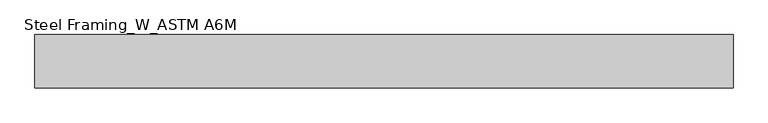
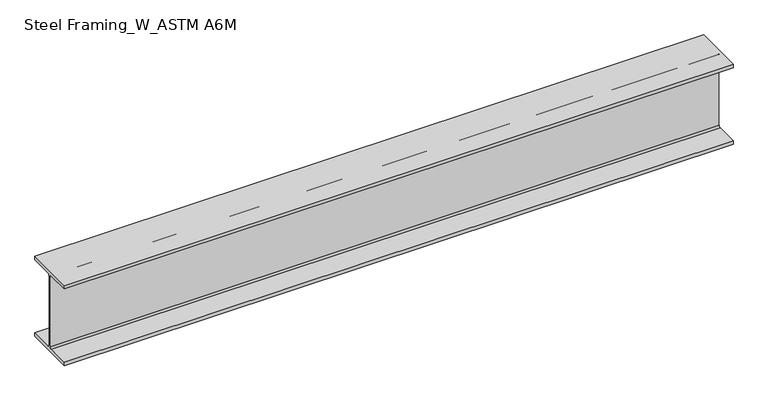
"""IFC4 building model written with IfcOpenShell, lengths in millimetres: beam geometry, Steel Framing_W_ASTM A6M : H_SB_AR_S02_W460x128_B1."""

import ifcopenshell
import ifcopenshell.guid

model = None  # the IFC model being written
_history = None  # IfcOwnerHistory: only IFC2X3 demands one
_inside = {}  # id of a spatial element -> (the spatial element, [elements in it])
_under = {}  # id of a project, library or spatial element -> (it, [spatial elements below it])
_declared = {}  # id of a project -> (the project, [libraries it declares])
_typed = {}  # id of a type object -> (the type object, [elements of that type])
_made_of = {}  # id of a material, layer set ... -> (it, [elements and type objects made of it])


def new_model(schema):
    """Start an empty IFC model of exactly this schema.

    Asked for "IFC4X3", IfcOpenShell would pick the latest addendum, in which some entities
    have other attributes; the version numbers below select the first issue.
    IFC2X3 requires an IfcOwnerHistory on every rooted entity: one is made here for all.
    """
    global model, _history
    if schema == "IFC4X3":
        model = ifcopenshell.file(schema_version=(4, 3, 0, 0))
    else:
        model = ifcopenshell.file(schema=schema)
    _inside.clear()
    _under.clear()
    _declared.clear()
    _typed.clear()
    _made_of.clear()
    _history = None
    if model.schema == "IFC2X3":
        org = make("IfcOrganization", Name="unknown")
        user = make(
            "IfcPersonAndOrganization",
            ThePerson=make("IfcPerson", FamilyName="unknown"),
            TheOrganization=org,
        )
        app = make(
            "IfcApplication",
            ApplicationDeveloper=org,
            Version="unknown",
            ApplicationFullName="unknown",
            ApplicationIdentifier="unknown",
        )
        _history = make(
            "IfcOwnerHistory",
            OwningUser=user,
            OwningApplication=app,
            ChangeAction="ADDED",
            CreationDate=0,
        )
    return model


def make(cls, **values):
    """One entity of the class cls with the attributes given. An attribute that is None is left unset."""
    return model.create_entity(
        cls, **{name: value for name, value in values.items() if value is not None}
    )


def rooted(cls, **values):
    """An entity with a GlobalId (a new one), such as an element, a storey or a relation."""
    return make(cls, GlobalId=ifcopenshell.guid.new(), OwnerHistory=_history, **values)


def si_unit(unit_type, name, prefix=None):
    """IfcSIUnit, for example si_unit("LENGTHUNIT", "METRE", prefix="MILLI")."""
    return make("IfcSIUnit", UnitType=unit_type, Prefix=prefix, Name=name)


def assignment(units):
    """IfcUnitAssignment: the units of a project."""
    return None if units is None else make("IfcUnitAssignment", Units=units)


def point(xyz):
    """IfcCartesianPoint."""
    return None if xyz is None else make("IfcCartesianPoint", Coordinates=xyz)


def direction(xyz):
    """IfcDirection."""
    return None if xyz is None else make("IfcDirection", DirectionRatios=xyz)


def frame(location, z_axis=None, x_axis=None):
    """IfcAxis2Placement3D, a coordinate frame: its origin and axes. An axis left out is left unset."""
    return make(
        "IfcAxis2Placement3D",
        Location=point(location),
        Axis=direction(z_axis),
        RefDirection=direction(x_axis),
    )


def frame_2d(location, x_axis=None):
    """IfcAxis2Placement2D, a coordinate frame in the plane: its origin and x axis."""
    return make(
        "IfcAxis2Placement2D", Location=point(location), RefDirection=direction(x_axis)
    )


def origin():
    """The frame at (0, 0, 0) with its axes left unset."""
    return frame((0.0, 0.0, 0.0))


def place(relative_to, where):
    """IfcLocalPlacement: puts the frame where relative to a parent placement (None: the world)."""
    return make(
        "IfcLocalPlacement", PlacementRelTo=relative_to, RelativePlacement=where
    )


def context(
    kind, dimensions, precision=None, world=None, true_north=None, identifier=None
):
    """IfcGeometricRepresentationContext, for example the 3D "Model" context."""
    return make(
        "IfcGeometricRepresentationContext",
        ContextIdentifier=identifier,
        ContextType=kind,
        CoordinateSpaceDimension=dimensions,
        Precision=precision,
        WorldCoordinateSystem=world,
        TrueNorth=true_north,
    )


def project(units=None, contexts=None):
    """IfcProject with its units and contexts."""
    return rooted(
        "IfcProject",
        Name="project",
        RepresentationContexts=contexts,
        UnitsInContext=assignment(units),
    )


def spatial(cls, under=None, at=None, **own):
    """A site, building, storey or space (cls), placed at a placement, below another one or the project."""
    s = rooted(cls, ObjectPlacement=at, **own)
    if under is not None:
        _under.setdefault(under.id(), (under, []))[1].append(s)
    return s


def polyline(points):
    """IfcPolyline through the points."""
    return make("IfcPolyline", Points=[point(p) for p in points])


def circle_curve(where, radius):
    """IfcCircle in the frame where."""
    return make("IfcCircle", Position=where, Radius=radius)


def trimmed(basis, trim1, trim2, sense, master):
    """IfcTrimmedCurve: the piece of a basis curve between two trims."""
    return make(
        "IfcTrimmedCurve",
        BasisCurve=basis,
        Trim1=trim1,
        Trim2=trim2,
        SenseAgreement=sense,
        MasterRepresentation=master,
    )


def segment(curve, same_sense, transition):
    """IfcCompositeCurveSegment."""
    return make(
        "IfcCompositeCurveSegment",
        Transition=transition,
        SameSense=same_sense,
        ParentCurve=curve,
    )


def composite_curve(segments, self_intersect=None):
    """IfcCompositeCurve: segments joined end to end."""
    return make("IfcCompositeCurve", Segments=segments, SelfIntersect=self_intersect)


def outline(outer, holes=None, kind="AREA"):
    """IfcArbitraryClosedProfileDef: a profile drawn as a closed curve; with holes, ...WithVoids."""
    if holes is None:
        return make("IfcArbitraryClosedProfileDef", ProfileType=kind, OuterCurve=outer)
    return make(
        "IfcArbitraryProfileDefWithVoids",
        ProfileType=kind,
        OuterCurve=outer,
        InnerCurves=holes,
    )


def extrude(swept, where, along, depth):
    """IfcExtrudedAreaSolid: the profile swept, set in the frame where, extruded along a direction by depth."""
    return make(
        "IfcExtrudedAreaSolid",
        SweptArea=swept,
        Position=where,
        ExtrudedDirection=direction(along),
        Depth=depth,
    )


def shape(context_of_items, identifier, shape_type, items):
    """IfcShapeRepresentation: the items that make up one representation, for example the "Body"."""
    return make(
        "IfcShapeRepresentation",
        ContextOfItems=context_of_items,
        RepresentationIdentifier=identifier,
        RepresentationType=shape_type,
        Items=items,
    )


def source(mapping_origin, context_of_items, identifier, shape_type, items):
    """IfcRepresentationMap: a shape defined once, which mapped items show again and again."""
    return make(
        "IfcRepresentationMap",
        MappingOrigin=mapping_origin,
        MappedRepresentation=shape(context_of_items, identifier, shape_type, items),
    )


def transform(
    local_origin,
    x_axis=None,
    y_axis=None,
    z_axis=None,
    scale=None,
    scale2=None,
    scale3=None,
    uniform=True,
):
    """IfcCartesianTransformationOperator3D, or its non-uniform kind. x_axis, y_axis, z_axis: its Axis1, 2, 3."""
    if uniform:
        return make(
            "IfcCartesianTransformationOperator3D",
            Axis1=direction(x_axis),
            Axis2=direction(y_axis),
            LocalOrigin=point(local_origin),
            Scale=scale,
            Axis3=direction(z_axis),
        )
    return make(
        "IfcCartesianTransformationOperator3DnonUniform",
        Axis1=direction(x_axis),
        Axis2=direction(y_axis),
        LocalOrigin=point(local_origin),
        Scale=scale,
        Axis3=direction(z_axis),
        Scale2=scale2,
        Scale3=scale3,
    )


def mapped(mapping_source, mapping_target):
    """IfcMappedItem: shows the shape of a source again, moved by a transform."""
    return make(
        "IfcMappedItem", MappingSource=mapping_source, MappingTarget=mapping_target
    )


def made_of(thing, what):
    """Note that an element or type object is made of a material, layer set ...; save() writes the relation."""
    if what is not None:
        _made_of.setdefault(what.id(), (what, []))[1].append(thing)
    return thing


def element(
    cls,
    number,
    at=None,
    inside=None,
    cuts=None,
    type_object=None,
    material=None,
    context=None,
    identifier="Body",
    shape_type=None,
    held_by="IfcProductDefinitionShape",
    body=None,
    shapes=None,
    **own,
):
    """One element of the class cls, such as IfcWall. Its Tag is "e" and its number.

    at: its placement. inside: the storey or other place that contains it. cuts: it is an
    opening in that element (IfcRelVoidsElement). A single representation is given by context,
    identifier, shape_type and body (its items); several are given by shapes. held_by: the class
    of the entity that holds the representations. save() writes the other relations.
    """
    e = rooted(cls, Tag="e%d" % number, ObjectPlacement=at, **own)
    if body is not None:
        shapes = [shape(context, identifier, shape_type, body)]
    if shapes is not None:
        e.Representation = make(held_by, Representations=shapes)
    if inside is not None:
        _inside.setdefault(inside.id(), (inside, []))[1].append(e)
    if cuts is not None:
        rooted(
            "IfcRelVoidsElement", RelatingBuildingElement=cuts, RelatedOpeningElement=e
        )
    if type_object is not None:
        _typed.setdefault(type_object.id(), (type_object, []))[1].append(e)
    return made_of(e, material)


def aggregate(whole, parts):
    """IfcRelAggregates: a whole, such as a stair, and the parts it consists of."""
    return rooted("IfcRelAggregates", RelatingObject=whole, RelatedObjects=parts)


def save(model, path):
    """Write the relations noted so far, then the file.

    IfcRelAggregates (storeys below a building ...), IfcRelContainedInSpatialStructure (elements
    in a storey), IfcRelDefinesByType, IfcRelAssociatesMaterial and IfcRelDeclares: one each for
    every whole, place, type object, material and project.
    """
    for whole, parts in _under.values():
        aggregate(whole, parts)
    for where, things in _inside.values():
        rooted(
            "IfcRelContainedInSpatialStructure",
            RelatedElements=things,
            RelatingStructure=where,
        )
    for kind, things in _typed.values():
        rooted("IfcRelDefinesByType", RelatedObjects=things, RelatingType=kind)
    for what, things in _made_of.values():
        rooted("IfcRelAssociatesMaterial", RelatedObjects=things, RelatingMaterial=what)
    for by, libraries in _declared.values():
        rooted("IfcRelDeclares", RelatingContext=by, RelatedDefinitions=libraries)
    model.write(path)


def steel_framing_w_astm_a6m_196e06da(model_context):
    return source(origin(), model_context, "Body", "SweptSolid", [
        extrude(outline(composite_curve([segment(polyline([(141.0, -213.9), (141.0, -233.5), (-141.0, -233.5), (-141.0, -213.9), (-16.2, -213.9)]), True, "CONTINUOUS"), segment(trimmed(circle_curve(frame_2d((-16.2, -203.8)), 10.1), [point((-16.2, -213.9))], [point((-6.1, -203.8))], True, "CARTESIAN"), True, "CONTINUOUS"), segment(polyline([(-6.1, -203.8), (-6.1, 203.8)]), True, "CONTINUOUS"), segment(trimmed(circle_curve(frame_2d((-16.2, 203.8)), 10.1), [point((-6.1, 203.8))], [point((-16.2, 213.9))], True, "CARTESIAN"), True, "CONTINUOUS"), segment(polyline([(-16.2, 213.9), (-141.0, 213.9), (-141.0, 233.5), (141.0, 233.5), (141.0, 213.9), (16.2, 213.9)]), True, "CONTINUOUS"), segment(trimmed(circle_curve(frame_2d((16.2, 203.8)), 10.1), [point((16.2, 213.9))], [point((6.1, 203.8))], True, "CARTESIAN"), True, "CONTINUOUS"), segment(polyline([(6.1, 203.8), (6.1, -203.8)]), True, "CONTINUOUS"), segment(trimmed(circle_curve(frame_2d((16.2, -203.8)), 10.1), [point((6.1, -203.8))], [point((16.2, -213.9))], True, "CARTESIAN"), True, "CONTINUOUS"), segment(polyline([(16.2, -213.9), (141.0, -213.9)]), True, "CONTINUOUS")], self_intersect=False)), frame((-1846.3, 0.0, 0.0), z_axis=(1.0, 0.0, 0.0), x_axis=(0.0, 1.0, 0.0)), (0.0, 0.0, 1.0), 3692.6),
    ])


if __name__ == "__main__":
    model = new_model("IFC4")
    model_context = context("Model", 3, world=origin())
    ifc_project = project(units=[si_unit("LENGTHUNIT", "METRE", prefix="MILLI")], contexts=[model_context])
    site = spatial("IfcSite", under=ifc_project)
    building = spatial("IfcBuilding", under=site)
    placement = place(None, origin())
    steel_framing_w_astm_a6m_shape = steel_framing_w_astm_a6m_196e06da(model_context)
    element("IfcBeam", 1, ObjectType="Steel Framing_W_ASTM A6M : H_SB_AR_S02_W460x128_B1", at=placement, inside=building, context=model_context, shape_type="MappedRepresentation", body=[
        mapped(steel_framing_w_astm_a6m_shape, transform((0.0, 0.0, 0.0), x_axis=(1.0, 0.0, 0.0), y_axis=(0.0, 1.0, 0.0), z_axis=(0.0, 0.0, 1.0))),
    ])
    save(model, "model.ifc")

# Revit data of these elements
# Type "Steel Framing_W_ASTM A6M : H_SB_AR_S02_W460x128_B1"
#   Section Name Key = "W18x86"
#   Width = 28.2 cm
#   Web Thickness = 1.22 cm
#   Web Fillet = 1.01 cm
#   Warping Constant = 3650000.0 cm⁶
#   Torsional Moment of Inertia = 171.00 cm⁴
#   Section Area = 163.0 cm²
#   Plastic Modulus weak axis = 793.0 cm³
#   Plastic Modulus strong axis = 3050.0 cm³
#   Perimeter = 2.02 m²/m
#   Nominal Weight = 128.00 kgf/m
#   Moment of Inertia weak axis = 7280.00 cm⁴
#   Moment of Inertia strong axis = 63700.00 cm⁴
#   Height = 46.7 cm
#   Flange Thickness = 1.96 cm
#   Elastic Modulus weak axis = 518.0 cm³
#   Elastic Modulus strong axis = 2720.0 cm³
#   Centroid Vertical = 23.35 cm
#   Centroid Horizontal = 14.1 cm
#   Length [instance default] = 1500 mm
#   Structural Material [instance default] = Steel, 45-345
#   Bolt Spacing = 0
#   Assembly Code = ""
# Element 1 (IfcBeam, "Steel Framing_W_ASTM A6M : H_SB_AR_S02_W460x128_B1")
#   Materials on its faces: "Steel, 45-345"
# Materials
#   "Steel, 45-345": class "Metal", colour RGB 189 187 185, transparency 0, Description = "Steel 345 MPa", Cost = 0
